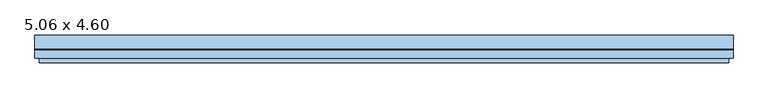
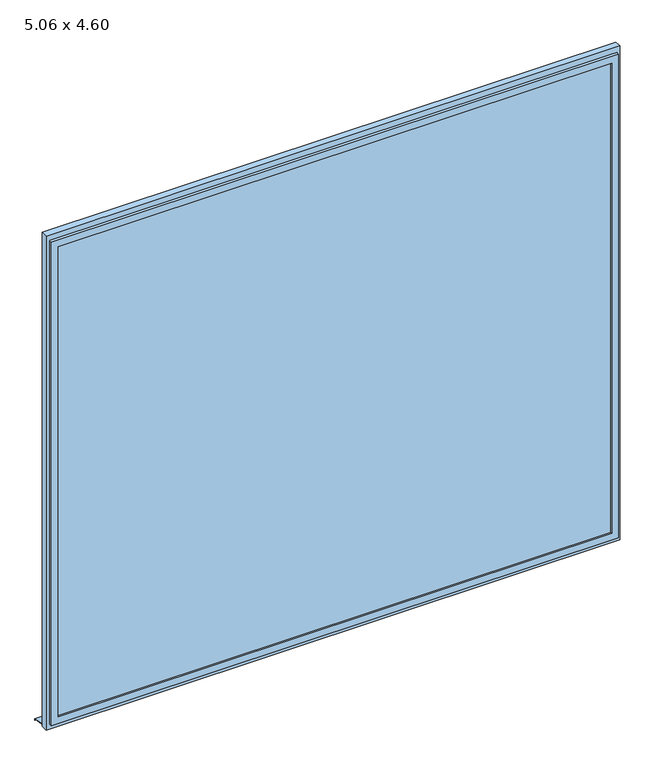
"""IFC4 building model written with IfcOpenShell, lengths in millimetres: window geometry, Fenstertür 1-flg : 5.06 x 4.60."""

from ifc_helpers import new_model, si_unit, frame, origin, place, context, project, spatial, polyline, outline, extrude, faceted_brep, source, transform, mapped, element, save


def window_5_06_x_4_60_7ceca0fc(model_context):
    return source(origin(), model_context, "Body", "SolidModel", [
        extrude(outline(polyline([(4600.0, 2530.0), (4600.0, -2530.0), (0.0, -2530.0), (0.0, 2530.0), (4600.0, 2530.0)]), holes=[polyline([(4520.0, 2470.0), (80.0, 2470.0), (80.0, -2470.0), (4520.0, -2470.0), (4520.0, 2470.0)])]), frame((0.0, -80.0, 0.0), z_axis=(0.0, 1.0, 0.0), x_axis=(0.0, 0.0, 1.0)), (0.0, 0.0, 1.0), 60.0),
        faceted_brep([(2500.0, -80.0, 4550.0), (2500.0, -110.0, 4550.0), (2500.0, -110.0, 50.0), (2500.0, -80.0, 50.0), (-2500.0, -110.0, 4550.0), (-2500.0, -110.0, 50.0), (2440.0, -110.0, 110.0), (-2440.0, -110.0, 110.0), (-2440.0, -110.0, 4490.0), (2440.0, -110.0, 4490.0), (-2500.0, -80.0, 50.0), (-2500.0, -80.0, 4550.0), (2470.0, -80.0, 4520.0), (-2470.0, -80.0, 4520.0), (-2470.0, -80.0, 80.0), (2470.0, -80.0, 80.0), (2470.0, -50.0, 4520.0), (2470.0, -50.0, 80.0), (-2470.0, -50.0, 80.0), (-2470.0, -50.0, 4520.0), (2440.0, -50.0, 4490.0), (-2440.0, -50.0, 4490.0), (-2440.0, -50.0, 110.0), (2440.0, -50.0, 110.0)], [[[0, 1, 2, 3]], [[1, 4, 5, 2], [6, 7, 8, 9]], [[3, 2, 5, 10]], [[3, 10, 11, 0], [12, 13, 14, 15]], [[16, 12, 15, 17]], [[17, 15, 14, 18]], [[17, 18, 19, 16], [20, 21, 22, 23]], [[9, 20, 23, 6]], [[6, 23, 22, 7]], [[10, 5, 4, 11]], [[18, 14, 13, 19]], [[7, 22, 21, 8]], [[11, 4, 1, 0]], [[19, 13, 12, 16]], [[8, 21, 20, 9]]]),
        extrude(outline(polyline([(-9.9778457, 20.0), (90.0, 0.0), (90.0, -10.0), (88.0, -10.0), (88.0, -1.6395366), (-10.1759277, 18.0), (-20.0, 18.0), (-20.0, 20.0), (-9.9778457, 20.0)])), frame((-2530.0, 0.0, 0.0), z_axis=(1.0, 0.0, 0.0), x_axis=(0.0, 1.0, 0.0)), (0.0, 0.0, 1.0), 5060.0),
        extrude(outline(polyline([(2440.0, -95.0), (-2440.0, -95.0), (-2440.0, -65.0), (2440.0, -65.0), (2440.0, -95.0)])), frame((0.0, 0.0, 110.0), z_axis=(0.0, 0.0, 1.0), x_axis=(1.0, 0.0, 0.0)), (0.0, 0.0, 1.0), 4380.0),
    ])


if __name__ == "__main__":
    model = new_model("IFC4")
    model_context = context("Model", 3, world=origin())
    ifc_project = project(units=[si_unit("LENGTHUNIT", "METRE", prefix="MILLI")], contexts=[model_context])
    site = spatial("IfcSite", under=ifc_project)
    building = spatial("IfcBuilding", under=site)
    placement = place(None, origin())
    window_5_06_x_4_60_shape = window_5_06_x_4_60_7ceca0fc(model_context)
    element("IfcWindow", 1, ObjectType="Fenstertür 1-flg : 5.06 x 4.60", at=placement, inside=building, context=model_context, shape_type="MappedRepresentation", body=[
        mapped(window_5_06_x_4_60_shape, transform((0.0, 0.0, 0.0), x_axis=(1.0, 0.0, 0.0), y_axis=(0.0, 1.0, 0.0), z_axis=(0.0, 0.0, 1.0))),
    ])
    save(model, "model.ifc")

# Revit data of these elements
# Type "Fenstertür 1-flg : 5.06 x 4.60"
#   Type Mark = "52"
#   Operation = "SinglePanel"
#   Construction Type Id = "SGL"
#   Keynote = "16.05.01"
#   Analytic Construction = "Große Fenster mit Einfachverglasung"
#   Visual Light Transmittance = 0.9
#   Solar Heat Gain Coefficient = 0.86
#   Rough Width = 5.060 m
#   Rough Height = 4.600 m
#   Heat Transfer Coefficient (U) = 5.5617 W/(m²·K)
#   Rahmentiefe = 0.060 m
#   Rahmenhöhe unten = 0.080 m
#   Höhe oberer  Rahmen = 0.080 m
#   Rahmenbreite = 0.060 m
#   Height = 4.600 m
#   Tiefe Flügel = 0.060 m
#   Flügelbreite = 0.060 m
#   Einbautiefe (von außen) [instance default] = 0.080 m
#   Width = 5.060 m
#   Sichtbarkeit Sturzlinien [instance default] = yes
#   Öffnungsrichtung oben [instance default] = yes
#   Öffnungsrichtung in Draufsicht anzeigen [instance default] = yes
#   Drehflügel 1 [instance default] = yes
#   Bild [instance default] = none
#   Glas [instance default] = none
#   Fensterflügel [instance default] = none
#   Äußere Fensterbank [instance default] = none
#   Wall Closure = (empty or 0)
# Element 1 (IfcWindow, "Fenstertür 1-flg : 5.06 x 4.60")
#   Materials on its faces: "Kunststoff - Weiß", "Glas"
# Materials
#   "Kunststoff - Weiß": class "Kunststoff", colour RGB 249 249 249, transparency 0, Cost = 0
#   "Glas": class "Glas", colour RGB 0 0 255, transparency 0.75, Comments = "Render-Darstellung nicht aktualisiert ", Cost = 0
